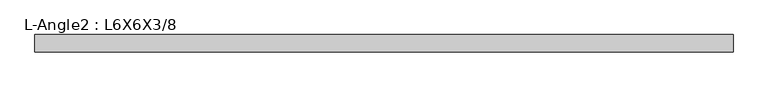
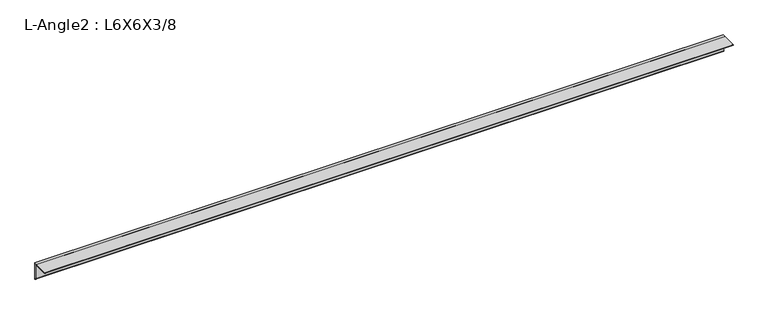
"""IFC4 building model written with IfcOpenShell, lengths in millimetres: member geometry, L-Angle2 : L6X6X3/8."""

from ifc_helpers import new_model, si_unit, point, frame, frame_2d, origin, place, context, project, spatial, polyline, circle_curve, trimmed, segment, composite_curve, outline, extrude, source, transform, mapped, element, save


def l_angle2_l6x6x3_8_edb1527c(model_context):
    return source(origin(), model_context, "Body", "SweptSolid", [
        extrude(outline(composite_curve([segment(polyline([(41.148, 41.148), (41.148, -111.252)]), True, "CONTINUOUS"), segment(trimmed(circle_curve(frame_2d((41.148, -101.727)), 9.525), [point((41.148, -111.252))], [point((31.623, -101.727))], False, "CARTESIAN"), True, "CONTINUOUS"), segment(polyline([(31.623, -101.727), (31.623, 22.098)]), True, "CONTINUOUS"), segment(trimmed(circle_curve(frame_2d((22.098, 22.098)), 9.525), [point((31.623, 22.098))], [point((22.098, 31.623))], True, "CARTESIAN"), True, "CONTINUOUS"), segment(polyline([(22.098, 31.623), (-101.727, 31.623)]), True, "CONTINUOUS"), segment(trimmed(circle_curve(frame_2d((-101.727, 41.148)), 9.525), [point((-101.727, 31.623))], [point((-111.252, 41.148))], False, "CARTESIAN"), True, "CONTINUOUS"), segment(polyline([(-111.252, 41.148), (41.148, 41.148)]), True, "CONTINUOUS")], self_intersect=False)), frame((-3087.7876533, 0.0, 0.0), z_axis=(1.0, 0.0, 0.0), x_axis=(0.0, 1.0, 0.0)), (0.0, 0.0, 1.0), 6141.9768896),
    ])


if __name__ == "__main__":
    model = new_model("IFC4")
    model_context = context("Model", 3, world=origin())
    ifc_project = project(units=[si_unit("LENGTHUNIT", "METRE", prefix="MILLI")], contexts=[model_context])
    site = spatial("IfcSite", under=ifc_project)
    building = spatial("IfcBuilding", under=site)
    placement = place(None, origin())
    l_angle2_l6x6x3_8_shape = l_angle2_l6x6x3_8_edb1527c(model_context)
    element("IfcMember", 1, ObjectType="L-Angle2 : L6X6X3/8", at=placement, inside=building, context=model_context, shape_type="MappedRepresentation", body=[
        mapped(l_angle2_l6x6x3_8_shape, transform((0.0, 0.0, 0.0), x_axis=(1.0, 0.0, 0.0), y_axis=(0.0, 1.0, 0.0), z_axis=(0.0, 0.0, 1.0))),
    ])
    save(model, "model.ifc")

# Revit data of these elements
# Type "L-Angle2 : L6X6X3/8"
#   Assembly Code = "B10"
#   k = 0' - 0 7/8"
#   W = 14.9
#   Length [instance default] = 5' - 0"
#   b = 0' - 6"
#   d = 0' - 6"
#   t = 0' - 0 3/8"
#   x = 0' - 1.62"
#   y = 0' - 1.62"
#   A = 0.0304167 SF
#   Structural Material [instance default] = Steel ASTM A36
# Element 1 (IfcMember, "L-Angle2 : L6X6X3/8")
#   Materials on its faces: "Steel ASTM A36"
# Materials
#   "Steel ASTM A36": class "Metal", colour RGB 199 199 199, transparency 0, Description = "Structural steel, ASTM A36 Grade B, mill finish", Cost = 0
